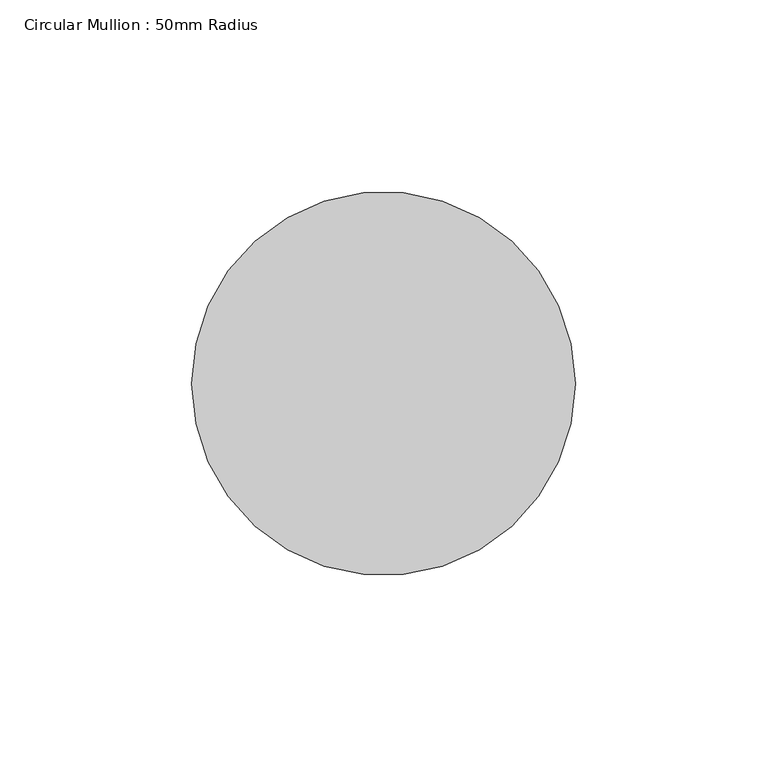
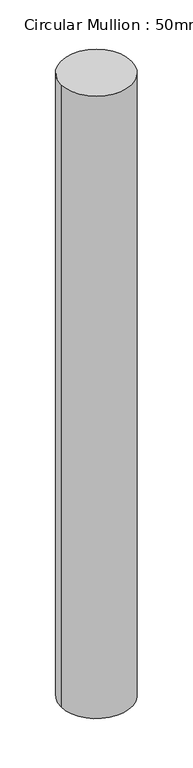
"""IFC4 building model written with IfcOpenShell, lengths in millimetres: member geometry, Circular Mullion : 50mm Radius."""

from ifc_helpers import new_model, si_unit, point, frame, origin, origin_2d, place, context, project, spatial, circle_curve, trimmed, segment, composite_curve, outline, extrude, source, transform, mapped, element, save


def circular_mullion_50mm_radius_df4fa90c(model_context):
    return source(origin(), model_context, "Body", "SweptSolid", [
        extrude(outline(composite_curve([segment(trimmed(circle_curve(origin_2d(), 50.0), [point((50.0, 0.0))], [point((-50.0, 0.0))], False, "CARTESIAN"), True, "CONTINUOUS"), segment(trimmed(circle_curve(origin_2d(), 50.0), [point((-50.0, 0.0))], [point((50.0, 0.0))], False, "CARTESIAN"), True, "CONTINUOUS")], self_intersect=False)), frame((0.0, 0.0, -930.4716735), z_axis=(0.0, 0.0, 1.0), x_axis=(1.0, 0.0, 0.0)), (0.0, 0.0, 1.0), 930.4716735),
    ])


if __name__ == "__main__":
    model = new_model("IFC4")
    model_context = context("Model", 3, world=origin())
    ifc_project = project(units=[si_unit("LENGTHUNIT", "METRE", prefix="MILLI")], contexts=[model_context])
    site = spatial("IfcSite", under=ifc_project)
    building = spatial("IfcBuilding", under=site)
    placement = place(None, origin())
    circular_mullion_50mm_radius_shape = circular_mullion_50mm_radius_df4fa90c(model_context)
    element("IfcMember", 1, ObjectType="Circular Mullion : 50mm Radius", at=placement, inside=building, context=model_context, shape_type="MappedRepresentation", body=[
        mapped(circular_mullion_50mm_radius_shape, transform((0.0, 0.0, 0.0), x_axis=(1.0, 0.0, 0.0), y_axis=(0.0, 1.0, 0.0), z_axis=(0.0, 0.0, 1.0))),
    ])
    save(model, "model.ifc")

# Revit data of these elements
# Type "Circular Mullion : 50mm Radius"
#   built-in parameter 1007350 = 0.164042 (stored number, unit not read)
# Element 1 (IfcMember, "Circular Mullion : 50mm Radius")
#   Materials on its faces: "Aluminium"
# Materials
#   "Aluminium": class "Metal", colour RGB 247 247 247, transparency 0, Description = "Aluminium 6061", Cost = 0
